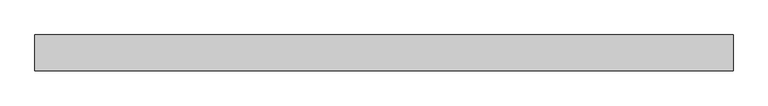
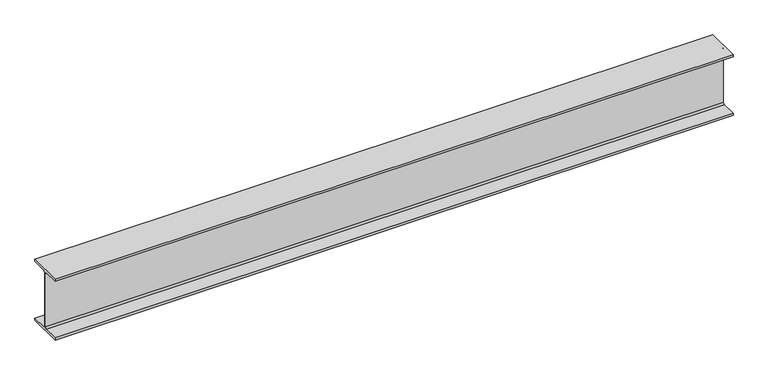
"""IFC4 building model written with IfcOpenShell, lengths in millimetres: beam geometry, Old_Steel Beam_H-KSD3502 : H_SB_ASB_H-200×200x8x12."""

from ifc_helpers import new_model, si_unit, point, frame, frame_2d, origin, place, context, project, spatial, polyline, circle_curve, trimmed, segment, composite_curve, outline, extrude, source, transform, mapped, element, save


def beam_058fccc5(model_context):
    return source(origin(), model_context, "Body", "SweptSolid", [
        extrude(outline(composite_curve([segment(polyline([(82.5, -141.5), (82.5, -151.7), (-82.5, -151.7), (-82.5, -141.5), (-11.9, -141.5)]), True, "CONTINUOUS"), segment(trimmed(circle_curve(frame_2d((-11.9, -132.6)), 8.9), [point((-11.9, -141.5))], [point((-3.0, -132.6))], True, "CARTESIAN"), True, "CONTINUOUS"), segment(polyline([(-3.0, -132.6), (-3.0, 132.6)]), True, "CONTINUOUS"), segment(trimmed(circle_curve(frame_2d((-11.9, 132.6)), 8.9), [point((-3.0, 132.6))], [point((-11.9, 141.5))], True, "CARTESIAN"), True, "CONTINUOUS"), segment(polyline([(-11.9, 141.5), (-82.5, 141.5), (-82.5, 151.7), (82.5, 151.7), (82.5, 141.5), (11.9, 141.5)]), True, "CONTINUOUS"), segment(trimmed(circle_curve(frame_2d((11.9, 132.6)), 8.9), [point((11.9, 141.5))], [point((3.0, 132.6))], True, "CARTESIAN"), True, "CONTINUOUS"), segment(polyline([(3.0, 132.6), (3.0, -132.6)]), True, "CONTINUOUS"), segment(trimmed(circle_curve(frame_2d((11.9, -132.6)), 8.9), [point((3.0, -132.6))], [point((11.9, -141.5))], True, "CARTESIAN"), True, "CONTINUOUS"), segment(polyline([(11.9, -141.5), (82.5, -141.5)]), True, "CONTINUOUS")], self_intersect=False)), frame((-1563.5376228, 0.0, 0.0), z_axis=(1.0, 0.0, 0.0), x_axis=(0.0, 1.0, 0.0)), (0.0, 0.0, 1.0), 3211.1247957),
    ])


if __name__ == "__main__":
    model = new_model("IFC4")
    model_context = context("Model", 3, world=origin())
    ifc_project = project(units=[si_unit("LENGTHUNIT", "METRE", prefix="MILLI")], contexts=[model_context])
    site = spatial("IfcSite", under=ifc_project)
    building = spatial("IfcBuilding", under=site)
    placement = place(None, origin())
    beam_shape = beam_058fccc5(model_context)
    element("IfcBeam", 1, ObjectType="Old_Steel Beam_H-KSD3502 : H_SB_ASB_H-200×200x8x12", at=placement, inside=building, context=model_context, shape_type="MappedRepresentation", body=[
        mapped(beam_shape, transform((0.0, 0.0, 0.0), x_axis=(1.0, 0.0, 0.0), y_axis=(0.0, 1.0, 0.0), z_axis=(0.0, 0.0, 1.0))),
    ])
    save(model, "model.ifc")

# Revit data of these elements
# Type "Old_Steel Beam_H-KSD3502 : H_SB_ASB_H-200×200x8x12"
#   Width = 20.0 cm
#   Web Thickness = 0.8 cm
#   Web Fillet = 1.3 cm
#   Warping Constant = 141376.0 cm⁶
#   Torsional Moment of Inertia = 26.2485 cm⁴
#   Torsional Modulus = 1.0 cm³
#   Section Area = 63.53 cm²
#   Plastic Modulus weak axis = 244.0 cm³
#   Plastic Modulus strong axis = 525.0 cm³
#   Perimeter = 1.16 m²/m
#   Nominal Weight = 49.90 kgf/m
#   Moment of Inertia weak axis = 1600.00 cm⁴
#   Moment of Inertia strong axis = 4720.00 cm⁴
#   Height = 20.0 cm
#   Flange Thickness = 1.2 cm
#   Elastic Modulus weak axis = 160.0 cm³
#   Elastic Modulus strong axis = 472.0 cm³
#   Centroid Vertical = 10.0 cm
#   Centroid Horizontal = 10.0 cm
#   Length [instance default] = 1.5240 m
#   Structural Material [instance default] = Steel, 45-345
#   Assembly Code = ""
# Element 1 (IfcBeam, "Old_Steel Beam_H-KSD3502 : H_SB_ASB_H-200×200x8x12")
#   Structural Material = none
# Materials
#   "Steel, 45-345": class "Metal", colour RGB 189 187 185, transparency 0, Description = "Steel 345 MPa", Cost = 0
